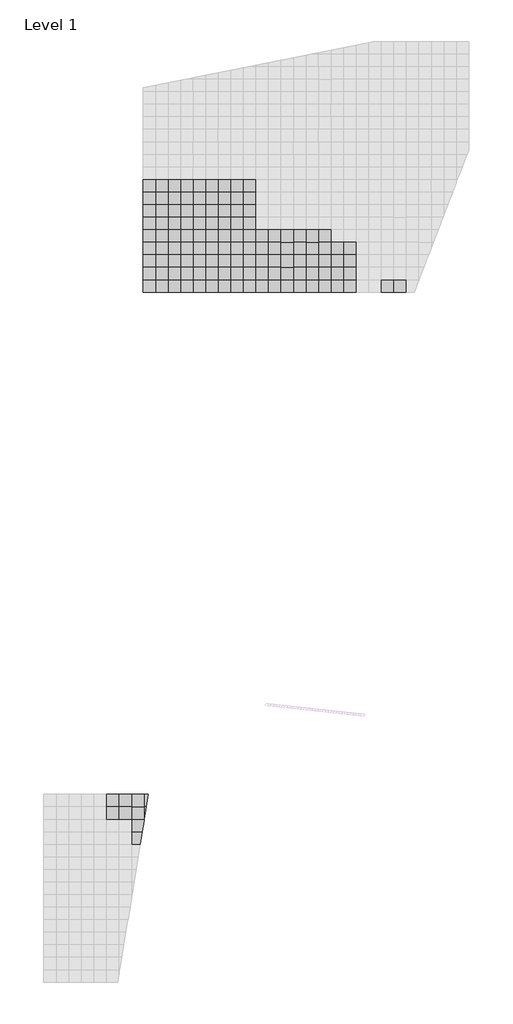
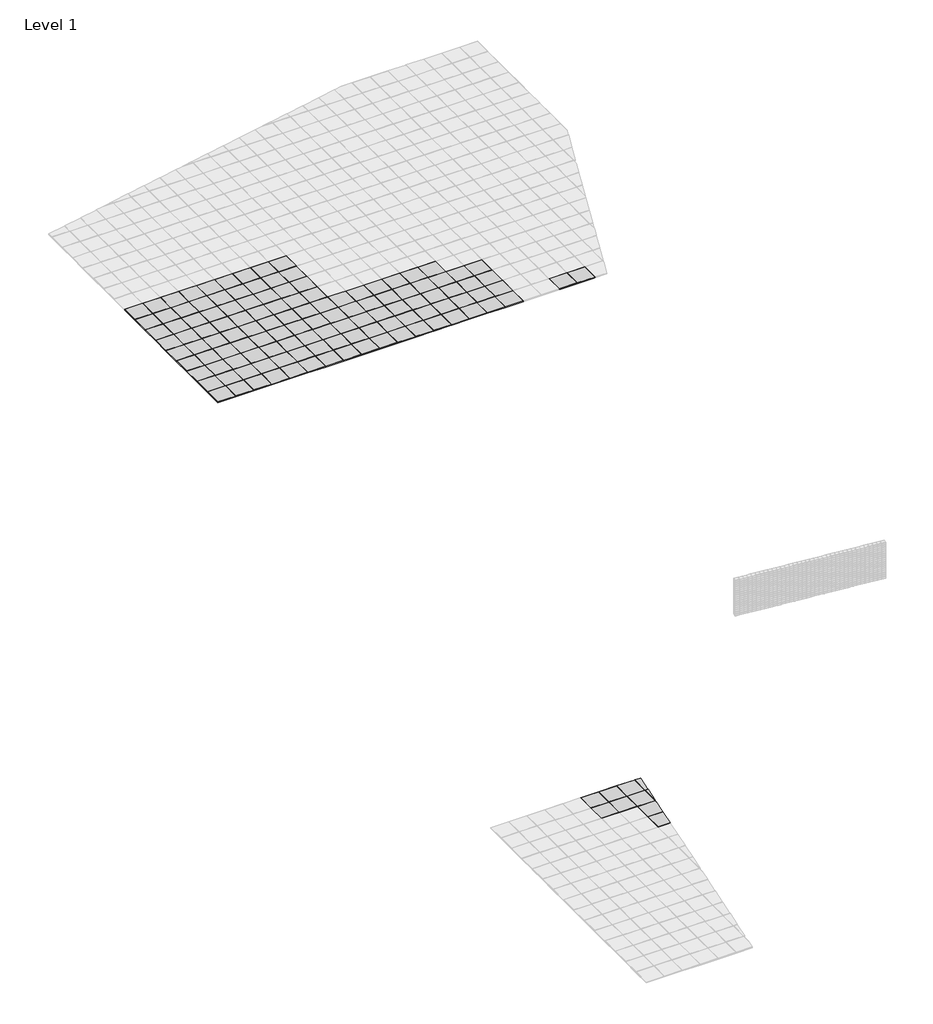
# One storey, part 3 of 18: 131 plates.
"""IFC4 building model written with IfcOpenShell, lengths in millimetres."""

import ifcopenshell
import ifcopenshell.guid

model = None  # the IFC model being written
_history = None  # IfcOwnerHistory: only IFC2X3 demands one
_inside = {}  # id of a spatial element -> (the spatial element, [elements in it])
_under = {}  # id of a project, library or spatial element -> (it, [spatial elements below it])
_declared = {}  # id of a project -> (the project, [libraries it declares])
_typed = {}  # id of a type object -> (the type object, [elements of that type])
_made_of = {}  # id of a material, layer set ... -> (it, [elements and type objects made of it])


def new_model(schema):
    """Start an empty IFC model of exactly this schema.

    Asked for "IFC4X3", IfcOpenShell would pick the latest addendum, in which some entities
    have other attributes; the version numbers below select the first issue.
    IFC2X3 requires an IfcOwnerHistory on every rooted entity: one is made here for all.
    """
    global model, _history
    if schema == "IFC4X3":
        model = ifcopenshell.file(schema_version=(4, 3, 0, 0))
    else:
        model = ifcopenshell.file(schema=schema)
    _inside.clear()
    _under.clear()
    _declared.clear()
    _typed.clear()
    _made_of.clear()
    _history = None
    if model.schema == "IFC2X3":
        org = make("IfcOrganization", Name="unknown")
        user = make(
            "IfcPersonAndOrganization",
            ThePerson=make("IfcPerson", FamilyName="unknown"),
            TheOrganization=org,
        )
        app = make(
            "IfcApplication",
            ApplicationDeveloper=org,
            Version="unknown",
            ApplicationFullName="unknown",
            ApplicationIdentifier="unknown",
        )
        _history = make(
            "IfcOwnerHistory",
            OwningUser=user,
            OwningApplication=app,
            ChangeAction="ADDED",
            CreationDate=0,
        )
    return model


def make(cls, **values):
    """One entity of the class cls with the attributes given. An attribute that is None is left unset."""
    return model.create_entity(
        cls, **{name: value for name, value in values.items() if value is not None}
    )


def rooted(cls, **values):
    """An entity with a GlobalId (a new one), such as an element, a storey or a relation."""
    return make(cls, GlobalId=ifcopenshell.guid.new(), OwnerHistory=_history, **values)


def si_unit(unit_type, name, prefix=None):
    """IfcSIUnit, for example si_unit("LENGTHUNIT", "METRE", prefix="MILLI")."""
    return make("IfcSIUnit", UnitType=unit_type, Prefix=prefix, Name=name)


def assignment(units):
    """IfcUnitAssignment: the units of a project."""
    return None if units is None else make("IfcUnitAssignment", Units=units)


def point(xyz):
    """IfcCartesianPoint."""
    return None if xyz is None else make("IfcCartesianPoint", Coordinates=xyz)


def direction(xyz):
    """IfcDirection."""
    return None if xyz is None else make("IfcDirection", DirectionRatios=xyz)


def frame(location, z_axis=None, x_axis=None):
    """IfcAxis2Placement3D, a coordinate frame: its origin and axes. An axis left out is left unset."""
    return make(
        "IfcAxis2Placement3D",
        Location=point(location),
        Axis=direction(z_axis),
        RefDirection=direction(x_axis),
    )


def origin():
    """The frame at (0, 0, 0) with its axes left unset."""
    return frame((0.0, 0.0, 0.0))


def origin_with_axes():
    """The frame at (0, 0, 0) with the z axis (0, 0, 1) and the x axis (1, 0, 0) written out."""
    return frame((0.0, 0.0, 0.0), z_axis=(0.0, 0.0, 1.0), x_axis=(1.0, 0.0, 0.0))


def place(relative_to, where):
    """IfcLocalPlacement: puts the frame where relative to a parent placement (None: the world)."""
    return make(
        "IfcLocalPlacement", PlacementRelTo=relative_to, RelativePlacement=where
    )


def context(
    kind, dimensions, precision=None, world=None, true_north=None, identifier=None
):
    """IfcGeometricRepresentationContext, for example the 3D "Model" context."""
    return make(
        "IfcGeometricRepresentationContext",
        ContextIdentifier=identifier,
        ContextType=kind,
        CoordinateSpaceDimension=dimensions,
        Precision=precision,
        WorldCoordinateSystem=world,
        TrueNorth=true_north,
    )


def project(units=None, contexts=None):
    """IfcProject with its units and contexts."""
    return rooted(
        "IfcProject",
        Name="project",
        RepresentationContexts=contexts,
        UnitsInContext=assignment(units),
    )


def spatial(cls, under=None, at=None, **own):
    """A site, building, storey or space (cls), placed at a placement, below another one or the project."""
    s = rooted(cls, ObjectPlacement=at, **own)
    if under is not None:
        _under.setdefault(under.id(), (under, []))[1].append(s)
    return s


def polyline(points):
    """IfcPolyline through the points."""
    return make("IfcPolyline", Points=[point(p) for p in points])


def outline(outer, holes=None, kind="AREA"):
    """IfcArbitraryClosedProfileDef: a profile drawn as a closed curve; with holes, ...WithVoids."""
    if holes is None:
        return make("IfcArbitraryClosedProfileDef", ProfileType=kind, OuterCurve=outer)
    return make(
        "IfcArbitraryProfileDefWithVoids",
        ProfileType=kind,
        OuterCurve=outer,
        InnerCurves=holes,
    )


def extrude(swept, where, along, depth):
    """IfcExtrudedAreaSolid: the profile swept, set in the frame where, extruded along a direction by depth."""
    return make(
        "IfcExtrudedAreaSolid",
        SweptArea=swept,
        Position=where,
        ExtrudedDirection=direction(along),
        Depth=depth,
    )


def shape(context_of_items, identifier, shape_type, items):
    """IfcShapeRepresentation: the items that make up one representation, for example the "Body"."""
    return make(
        "IfcShapeRepresentation",
        ContextOfItems=context_of_items,
        RepresentationIdentifier=identifier,
        RepresentationType=shape_type,
        Items=items,
    )


def source(mapping_origin, context_of_items, identifier, shape_type, items):
    """IfcRepresentationMap: a shape defined once, which mapped items show again and again."""
    return make(
        "IfcRepresentationMap",
        MappingOrigin=mapping_origin,
        MappedRepresentation=shape(context_of_items, identifier, shape_type, items),
    )


def transform(
    local_origin,
    x_axis=None,
    y_axis=None,
    z_axis=None,
    scale=None,
    scale2=None,
    scale3=None,
    uniform=True,
):
    """IfcCartesianTransformationOperator3D, or its non-uniform kind. x_axis, y_axis, z_axis: its Axis1, 2, 3."""
    if uniform:
        return make(
            "IfcCartesianTransformationOperator3D",
            Axis1=direction(x_axis),
            Axis2=direction(y_axis),
            LocalOrigin=point(local_origin),
            Scale=scale,
            Axis3=direction(z_axis),
        )
    return make(
        "IfcCartesianTransformationOperator3DnonUniform",
        Axis1=direction(x_axis),
        Axis2=direction(y_axis),
        LocalOrigin=point(local_origin),
        Scale=scale,
        Axis3=direction(z_axis),
        Scale2=scale2,
        Scale3=scale3,
    )


def mapped(mapping_source, mapping_target):
    """IfcMappedItem: shows the shape of a source again, moved by a transform."""
    return make(
        "IfcMappedItem", MappingSource=mapping_source, MappingTarget=mapping_target
    )


def made_of(thing, what):
    """Note that an element or type object is made of a material, layer set ...; save() writes the relation."""
    if what is not None:
        _made_of.setdefault(what.id(), (what, []))[1].append(thing)
    return thing


def element(
    cls,
    number,
    at=None,
    inside=None,
    cuts=None,
    type_object=None,
    material=None,
    context=None,
    identifier="Body",
    shape_type=None,
    held_by="IfcProductDefinitionShape",
    body=None,
    shapes=None,
    **own,
):
    """One element of the class cls, such as IfcWall. Its Tag is "e" and its number.

    at: its placement. inside: the storey or other place that contains it. cuts: it is an
    opening in that element (IfcRelVoidsElement). A single representation is given by context,
    identifier, shape_type and body (its items); several are given by shapes. held_by: the class
    of the entity that holds the representations. save() writes the other relations.
    """
    e = rooted(cls, Tag="e%d" % number, ObjectPlacement=at, **own)
    if body is not None:
        shapes = [shape(context, identifier, shape_type, body)]
    if shapes is not None:
        e.Representation = make(held_by, Representations=shapes)
    if inside is not None:
        _inside.setdefault(inside.id(), (inside, []))[1].append(e)
    if cuts is not None:
        rooted(
            "IfcRelVoidsElement", RelatingBuildingElement=cuts, RelatedOpeningElement=e
        )
    if type_object is not None:
        _typed.setdefault(type_object.id(), (type_object, []))[1].append(e)
    return made_of(e, material)


def aggregate(whole, parts):
    """IfcRelAggregates: a whole, such as a stair, and the parts it consists of."""
    return rooted("IfcRelAggregates", RelatingObject=whole, RelatedObjects=parts)


def save(model, path):
    """Write the relations noted so far, then the file.

    IfcRelAggregates (storeys below a building ...), IfcRelContainedInSpatialStructure (elements
    in a storey), IfcRelDefinesByType, IfcRelAssociatesMaterial and IfcRelDeclares: one each for
    every whole, place, type object, material and project.
    """
    for whole, parts in _under.values():
        aggregate(whole, parts)
    for where, things in _inside.values():
        rooted(
            "IfcRelContainedInSpatialStructure",
            RelatedElements=things,
            RelatingStructure=where,
        )
    for kind, things in _typed.values():
        rooted("IfcRelDefinesByType", RelatedObjects=things, RelatingType=kind)
    for what, things in _made_of.values():
        rooted("IfcRelAssociatesMaterial", RelatedObjects=things, RelatingMaterial=what)
    for by, libraries in _declared.values():
        rooted("IfcRelDeclares", RelatingContext=by, RelatedDefinitions=libraries)
    model.write(path)


def type_1_8eb2385c(model_context):
    return source(origin(), model_context, "Body", "SweptSolid", [
        extrude(outline(polyline([(1000.0, 500.0), (500.0, 500.0), (500.0, 1000.0), (1000.0, 1000.0), (1000.0, 500.0)]), holes=[polyline([(995.0, 995.0), (505.0, 995.0), (505.0, 505.0), (995.0, 505.0), (995.0, 995.0)])]), origin_with_axes(), (0.0, 0.0, 1.0), 18.0),
        extrude(outline(polyline([(505.0, 995.0), (995.0, 995.0), (995.0, 505.0), (505.0, 505.0), (505.0, 995.0)])), origin_with_axes(), (0.0, 0.0, 1.0), 20.0),
    ])


model = new_model("IFC4")

# Units and contexts
model_context = context("Model", 3, world=origin())
ifc_project = project(units=[si_unit("LENGTHUNIT", "METRE", prefix="MILLI")], contexts=[model_context])

# Site, building, storey
site = spatial("IfcSite", under=ifc_project)
building = spatial("IfcBuilding", under=site)
storey = spatial("IfcBuildingStorey", under=building, Name="Level 1", Elevation=0.0)

# Plates
placement = place(None, origin())
element("IfcPlate", 1, ObjectType="00_CPA_tegel : Type 1", at=placement, inside=storey, context=model_context, shape_type="SweptSolid", body=[
    extrude(outline(polyline([(3554.3495497, -9904.4739057), (3554.3593325, -9414.4739058), (3972.5227781, -9414.4822543), (3892.8479077, -9904.4806637), (3554.3495497, -9904.4739057)])), frame((0.0, 0.0, 1000.0), z_axis=(0.0, 0.0, 1.0), x_axis=(1.0, 0.0, 0.0)), (0.0, 0.0, 1.0), 20.0),
    extrude(outline(polyline([(3549.3494499, -9909.4738058), (3549.3594323, -9409.4738059), (3973.335787, -9409.4822706), (3972.5227781, -9414.4822543), (3554.3593325, -9414.4739058), (3554.3495497, -9904.4739057), (3892.8479077, -9904.4806637), (3892.0348989, -9909.4806475), (3549.3494499, -9909.4738058)])), frame((0.0, 0.0, 1000.0), z_axis=(0.0, 0.0, 1.0), x_axis=(1.0, 0.0, 0.0)), (0.0, 0.0, 1.0), 18.0),
])
element("IfcPlate", 2, ObjectType="00_CPA_tegel : Type 1", at=placement, inside=storey, context=model_context, shape_type="SweptSolid", body=[
    extrude(outline(polyline([(3554.3595321, -9404.4739058), (3554.3693149, -8914.4739059), (4044.3693148, -8914.4836887), (4044.3681538, -8972.6350365), (3974.1487959, -9404.4822868), (3554.3595321, -9404.4739058)])), frame((0.0, 0.0, 1000.0), z_axis=(0.0, 0.0, 1.0), x_axis=(1.0, 0.0, 0.0)), (0.0, 0.0, 1.0), 20.0),
    extrude(outline(polyline([(3549.3694147, -8909.473806), (4049.3694146, -8909.4837885), (4049.3687678, -8941.8813887), (4044.3681538, -8972.6350365), (4044.3693148, -8914.4836887), (3554.3693149, -8914.4739059), (3554.3595321, -9404.4739058), (3974.1487959, -9404.4822868), (3973.335787, -9409.4822706), (3549.3594323, -9409.4738059), (3549.3694147, -8909.473806)])), frame((0.0, 0.0, 1000.0), z_axis=(0.0, 0.0, 1.0), x_axis=(1.0, 0.0, 0.0)), (0.0, 0.0, 1.0), 18.0),
])
element("IfcPlate", 3, ObjectType="00_CPA_tegel : Type 1", at=placement, inside=storey, context=model_context, shape_type="SweptSolid", body=[
    extrude(outline(polyline([(3554.3695146, -8904.4739059), (3554.3792973, -8414.473906), (4044.3792972, -8414.4836888), (4044.3695145, -8904.4836887), (3554.3695146, -8904.4739059)])), frame((0.0, 0.0, 1000.0), z_axis=(0.0, 0.0, 1.0), x_axis=(1.0, 0.0, 0.0)), (0.0, 0.0, 1.0), 20.0),
    extrude(outline(polyline([(4049.3694146, -8909.4837885), (3549.3694147, -8909.473806), (3549.3793972, -8409.4738061), (4049.3793971, -8409.4837886), (4049.3694146, -8909.4837885)]), holes=[polyline([(4044.3792972, -8414.4836888), (3554.3792973, -8414.473906), (3554.3695146, -8904.4739059), (4044.3695145, -8904.4836887), (4044.3792972, -8414.4836888)])]), frame((0.0, 0.0, 1000.0), z_axis=(0.0, 0.0, 1.0), x_axis=(1.0, 0.0, 0.0)), (0.0, 0.0, 1.0), 18.0),
])
element("IfcPlate", 4, ObjectType="00_CPA_tegel : Type 1", at=placement, inside=storey, context=model_context, shape_type="SweptSolid", body=[
    extrude(outline(polyline([(4054.3695145, -8904.4838883), (4054.3792972, -8414.4838884), (4135.1245544, -8414.4855005), (4055.4496841, -8904.4839099), (4054.3695145, -8904.4838883)])), frame((0.0, 0.0, 1000.0), z_axis=(0.0, 0.0, 1.0), x_axis=(1.0, 0.0, 0.0)), (0.0, 0.0, 1.0), 20.0),
    extrude(outline(polyline([(4049.3694146, -8909.4837885), (4049.3793971, -8409.4837886), (4135.9375633, -8409.4855167), (4135.1245544, -8414.4855005), (4054.3792972, -8414.4838884), (4054.3695145, -8904.4838883), (4055.4496841, -8904.4839099), (4054.6366752, -8909.4838936), (4049.3694146, -8909.4837885)])), frame((0.0, 0.0, 1000.0), z_axis=(0.0, 0.0, 1.0), x_axis=(1.0, 0.0, 0.0)), (0.0, 0.0, 1.0), 18.0),
])
element("IfcPlate", 5, ObjectType="00_CPA_tegel : Type 1", at=placement, inside=storey, context=model_context, shape_type="SweptSolid", body=[
    extrude(outline(polyline([(4054.3794969, -8404.4838884), (4054.3892797, -7914.4838885), (4216.4254426, -7914.4871235), (4136.7505722, -8404.4855329), (4054.3794969, -8404.4838884)])), frame((0.0, 0.0, 1000.0), z_axis=(0.0, 0.0, 1.0), x_axis=(1.0, 0.0, 0.0)), (0.0, 0.0, 1.0), 20.0),
    extrude(outline(polyline([(4049.3793971, -8409.4837886), (4049.3893795, -7909.4837887), (4217.2384514, -7909.4871398), (4216.4254426, -7914.4871235), (4054.3892797, -7914.4838885), (4054.3794969, -8404.4838884), (4136.7505722, -8404.4855329), (4135.9375633, -8409.4855167), (4049.3793971, -8409.4837886)])), frame((0.0, 0.0, 1000.0), z_axis=(0.0, 0.0, 1.0), x_axis=(1.0, 0.0, 0.0)), (0.0, 0.0, 1.0), 18.0),
])
type_1_shape = type_1_8eb2385c(model_context)
element("IfcPlate", 6, ObjectType="00_CPA_tegel : Type 1", at=placement, inside=storey, context=model_context, shape_type="MappedRepresentation", body=[
    mapped(type_1_shape, transform((3506.2147669, 11592.7016515, 0.0), x_axis=(1.0000000000000002, 0.0, 0.0), y_axis=(0.0, 1.0000000000000002, 0.0), z_axis=(0.0, 0.0, 1.0))),
])
element("IfcPlate", 7, ObjectType="00_CPA_tegel : Type 1", at=placement, inside=storey, context=model_context, shape_type="MappedRepresentation", body=[
    mapped(type_1_shape, transform((4006.2147669, 11592.7016515, 0.0), x_axis=(1.0000000000000002, 0.0, 0.0), y_axis=(0.0, 1.0000000000000002, 0.0), z_axis=(0.0, 0.0, 1.0))),
])
element("IfcPlate", 8, ObjectType="00_CPA_tegel : Type 1", at=placement, inside=storey, context=model_context, shape_type="MappedRepresentation", body=[
    mapped(type_1_shape, transform((4506.2147669, 11592.7016515, 0.0), x_axis=(1.0000000000000002, 0.0, 0.0), y_axis=(0.0, 1.0000000000000002, 0.0), z_axis=(0.0, 0.0, 1.0))),
])
element("IfcPlate", 9, ObjectType="00_CPA_tegel : Type 1", at=placement, inside=storey, context=model_context, shape_type="MappedRepresentation", body=[
    mapped(type_1_shape, transform((5006.2147669, 11592.7016515, 0.0), x_axis=(1.0000000000000002, 0.0, 0.0), y_axis=(0.0, 1.0000000000000002, 0.0), z_axis=(0.0, 0.0, 1.0))),
])
element("IfcPlate", 10, ObjectType="00_CPA_tegel : Type 1", at=placement, inside=storey, context=model_context, shape_type="MappedRepresentation", body=[
    mapped(type_1_shape, transform((5506.2147669, 11592.7016515, 0.0), x_axis=(1.0000000000000002, 0.0, 0.0), y_axis=(0.0, 1.0000000000000002, 0.0), z_axis=(0.0, 0.0, 1.0))),
])
element("IfcPlate", 11, ObjectType="00_CPA_tegel : Type 1", at=placement, inside=storey, context=model_context, shape_type="MappedRepresentation", body=[
    mapped(type_1_shape, transform((6006.2147669, 11592.7016515, 0.0), x_axis=(1.0000000000000002, 0.0, 0.0), y_axis=(0.0, 1.0000000000000002, 0.0), z_axis=(0.0, 0.0, 1.0))),
])
element("IfcPlate", 12, ObjectType="00_CPA_tegel : Type 1", at=placement, inside=storey, context=model_context, shape_type="MappedRepresentation", body=[
    mapped(type_1_shape, transform((6506.2147669, 11592.7016515, 0.0), x_axis=(1.0000000000000002, 0.0, 0.0), y_axis=(0.0, 1.0000000000000002, 0.0), z_axis=(0.0, 0.0, 1.0))),
])
element("IfcPlate", 13, ObjectType="00_CPA_tegel : Type 1", at=placement, inside=storey, context=model_context, shape_type="MappedRepresentation", body=[
    mapped(type_1_shape, transform((7006.2147669, 11592.7016515, 0.0), x_axis=(1.0000000000000002, 0.0, 0.0), y_axis=(0.0, 1.0000000000000002, 0.0), z_axis=(0.0, 0.0, 1.0))),
])
element("IfcPlate", 14, ObjectType="00_CPA_tegel : Type 1", at=placement, inside=storey, context=model_context, shape_type="MappedRepresentation", body=[
    mapped(type_1_shape, transform((7506.2147669, 11592.7016515, 0.0), x_axis=(1.0000000000000002, 0.0, 0.0), y_axis=(0.0, 1.0000000000000002, 0.0), z_axis=(0.0, 0.0, 1.0))),
])
element("IfcPlate", 15, ObjectType="00_CPA_tegel : Type 1", at=placement, inside=storey, context=model_context, shape_type="MappedRepresentation", body=[
    mapped(type_1_shape, transform((3506.2147669, 12092.7016515, 0.0), x_axis=(1.0000000000000002, 0.0, 0.0), y_axis=(0.0, 1.0000000000000002, 0.0), z_axis=(0.0, 0.0, 1.0))),
])
element("IfcPlate", 16, ObjectType="00_CPA_tegel : Type 1", at=placement, inside=storey, context=model_context, shape_type="MappedRepresentation", body=[
    mapped(type_1_shape, transform((4006.2147669, 12092.7016515, 0.0), x_axis=(1.0000000000000002, 0.0, 0.0), y_axis=(0.0, 1.0000000000000002, 0.0), z_axis=(0.0, 0.0, 1.0))),
])
element("IfcPlate", 17, ObjectType="00_CPA_tegel : Type 1", at=placement, inside=storey, context=model_context, shape_type="MappedRepresentation", body=[
    mapped(type_1_shape, transform((4506.2147669, 12092.7016515, 0.0), x_axis=(1.0000000000000002, 0.0, 0.0), y_axis=(0.0, 1.0000000000000002, 0.0), z_axis=(0.0, 0.0, 1.0))),
])
element("IfcPlate", 18, ObjectType="00_CPA_tegel : Type 1", at=placement, inside=storey, context=model_context, shape_type="MappedRepresentation", body=[
    mapped(type_1_shape, transform((5006.2147669, 12092.7016515, 0.0), x_axis=(1.0000000000000002, 0.0, 0.0), y_axis=(0.0, 1.0000000000000002, 0.0), z_axis=(0.0, 0.0, 1.0))),
])
element("IfcPlate", 19, ObjectType="00_CPA_tegel : Type 1", at=placement, inside=storey, context=model_context, shape_type="MappedRepresentation", body=[
    mapped(type_1_shape, transform((5506.2147669, 12092.7016515, 0.0), x_axis=(1.0000000000000002, 0.0, 0.0), y_axis=(0.0, 1.0000000000000002, 0.0), z_axis=(0.0, 0.0, 1.0))),
])
element("IfcPlate", 20, ObjectType="00_CPA_tegel : Type 1", at=placement, inside=storey, context=model_context, shape_type="MappedRepresentation", body=[
    mapped(type_1_shape, transform((6006.2147669, 12092.7016515, 0.0), x_axis=(1.0000000000000002, 0.0, 0.0), y_axis=(0.0, 1.0000000000000002, 0.0), z_axis=(0.0, 0.0, 1.0))),
])
element("IfcPlate", 21, ObjectType="00_CPA_tegel : Type 1", at=placement, inside=storey, context=model_context, shape_type="MappedRepresentation", body=[
    mapped(type_1_shape, transform((6506.2147669, 12092.7016515, 0.0), x_axis=(1.0000000000000002, 0.0, 0.0), y_axis=(0.0, 1.0000000000000002, 0.0), z_axis=(0.0, 0.0, 1.0))),
])
element("IfcPlate", 22, ObjectType="00_CPA_tegel : Type 1", at=placement, inside=storey, context=model_context, shape_type="MappedRepresentation", body=[
    mapped(type_1_shape, transform((7006.2147669, 12092.7016515, 0.0), x_axis=(1.0000000000000002, 0.0, 0.0), y_axis=(0.0, 1.0000000000000002, 0.0), z_axis=(0.0, 0.0, 1.0))),
])
element("IfcPlate", 23, ObjectType="00_CPA_tegel : Type 1", at=placement, inside=storey, context=model_context, shape_type="MappedRepresentation", body=[
    mapped(type_1_shape, transform((7506.2147669, 12092.7016515, 0.0), x_axis=(1.0000000000000002, 0.0, 0.0), y_axis=(0.0, 1.0000000000000002, 0.0), z_axis=(0.0, 0.0, 1.0))),
])
element("IfcPlate", 24, ObjectType="00_CPA_tegel : Type 1", at=placement, inside=storey, context=model_context, shape_type="MappedRepresentation", body=[
    mapped(type_1_shape, transform((3506.2147669, 12592.7016515, 0.0), x_axis=(1.0000000000000002, 0.0, 0.0), y_axis=(0.0, 1.0000000000000002, 0.0), z_axis=(0.0, 0.0, 1.0))),
])
element("IfcPlate", 25, ObjectType="00_CPA_tegel : Type 1", at=placement, inside=storey, context=model_context, shape_type="MappedRepresentation", body=[
    mapped(type_1_shape, transform((4006.2147669, 12592.7016515, 0.0), x_axis=(1.0000000000000002, 0.0, 0.0), y_axis=(0.0, 1.0000000000000002, 0.0), z_axis=(0.0, 0.0, 1.0))),
])
element("IfcPlate", 26, ObjectType="00_CPA_tegel : Type 1", at=placement, inside=storey, context=model_context, shape_type="MappedRepresentation", body=[
    mapped(type_1_shape, transform((4506.2147669, 12592.7016515, 0.0), x_axis=(1.0000000000000002, 0.0, 0.0), y_axis=(0.0, 1.0000000000000002, 0.0), z_axis=(0.0, 0.0, 1.0))),
])
element("IfcPlate", 27, ObjectType="00_CPA_tegel : Type 1", at=placement, inside=storey, context=model_context, shape_type="MappedRepresentation", body=[
    mapped(type_1_shape, transform((5006.2147669, 12592.7016515, 0.0), x_axis=(1.0000000000000002, 0.0, 0.0), y_axis=(0.0, 1.0000000000000002, 0.0), z_axis=(0.0, 0.0, 1.0))),
])
element("IfcPlate", 28, ObjectType="00_CPA_tegel : Type 1", at=placement, inside=storey, context=model_context, shape_type="MappedRepresentation", body=[
    mapped(type_1_shape, transform((5506.2147669, 12592.7016515, 0.0), x_axis=(1.0000000000000002, 0.0, 0.0), y_axis=(0.0, 1.0000000000000002, 0.0), z_axis=(0.0, 0.0, 1.0))),
])
element("IfcPlate", 29, ObjectType="00_CPA_tegel : Type 1", at=placement, inside=storey, context=model_context, shape_type="MappedRepresentation", body=[
    mapped(type_1_shape, transform((6006.2147669, 12592.7016515, 0.0), x_axis=(1.0000000000000002, 0.0, 0.0), y_axis=(0.0, 1.0000000000000002, 0.0), z_axis=(0.0, 0.0, 1.0))),
])
element("IfcPlate", 30, ObjectType="00_CPA_tegel : Type 1", at=placement, inside=storey, context=model_context, shape_type="MappedRepresentation", body=[
    mapped(type_1_shape, transform((6506.2147669, 12592.7016515, 0.0), x_axis=(1.0000000000000002, 0.0, 0.0), y_axis=(0.0, 1.0000000000000002, 0.0), z_axis=(0.0, 0.0, 1.0))),
])
element("IfcPlate", 31, ObjectType="00_CPA_tegel : Type 1", at=placement, inside=storey, context=model_context, shape_type="MappedRepresentation", body=[
    mapped(type_1_shape, transform((7006.2147669, 12592.7016515, 0.0), x_axis=(1.0000000000000002, 0.0, 0.0), y_axis=(0.0, 1.0000000000000002, 0.0), z_axis=(0.0, 0.0, 1.0))),
])
element("IfcPlate", 32, ObjectType="00_CPA_tegel : Type 1", at=placement, inside=storey, context=model_context, shape_type="MappedRepresentation", body=[
    mapped(type_1_shape, transform((7506.2147669, 12592.7016515, 0.0), x_axis=(1.0000000000000002, 0.0, 0.0), y_axis=(0.0, 1.0000000000000002, 0.0), z_axis=(0.0, 0.0, 1.0))),
])
element("IfcPlate", 33, ObjectType="00_CPA_tegel : Type 1", at=placement, inside=storey, context=model_context, shape_type="MappedRepresentation", body=[
    mapped(type_1_shape, transform((3506.2147669, 13092.7016515, 0.0), x_axis=(1.0000000000000002, 0.0, 0.0), y_axis=(0.0, 1.0000000000000002, 0.0), z_axis=(0.0, 0.0, 1.0))),
])
element("IfcPlate", 34, ObjectType="00_CPA_tegel : Type 1", at=placement, inside=storey, context=model_context, shape_type="MappedRepresentation", body=[
    mapped(type_1_shape, transform((4006.2147669, 13092.7016515, 0.0), x_axis=(1.0000000000000002, 0.0, 0.0), y_axis=(0.0, 1.0000000000000002, 0.0), z_axis=(0.0, 0.0, 1.0))),
])
element("IfcPlate", 35, ObjectType="00_CPA_tegel : Type 1", at=placement, inside=storey, context=model_context, shape_type="MappedRepresentation", body=[
    mapped(type_1_shape, transform((4506.2147669, 13092.7016515, 0.0), x_axis=(1.0000000000000002, 0.0, 0.0), y_axis=(0.0, 1.0000000000000002, 0.0), z_axis=(0.0, 0.0, 1.0))),
])
element("IfcPlate", 36, ObjectType="00_CPA_tegel : Type 1", at=placement, inside=storey, context=model_context, shape_type="MappedRepresentation", body=[
    mapped(type_1_shape, transform((5006.2147669, 13092.7016515, 0.0), x_axis=(1.0000000000000002, 0.0, 0.0), y_axis=(0.0, 1.0000000000000002, 0.0), z_axis=(0.0, 0.0, 1.0))),
])
element("IfcPlate", 37, ObjectType="00_CPA_tegel : Type 1", at=placement, inside=storey, context=model_context, shape_type="MappedRepresentation", body=[
    mapped(type_1_shape, transform((5506.2147669, 13092.7016515, 0.0), x_axis=(1.0000000000000002, 0.0, 0.0), y_axis=(0.0, 1.0000000000000002, 0.0), z_axis=(0.0, 0.0, 1.0))),
])
element("IfcPlate", 38, ObjectType="00_CPA_tegel : Type 1", at=placement, inside=storey, context=model_context, shape_type="MappedRepresentation", body=[
    mapped(type_1_shape, transform((6006.2147669, 13092.7016515, 0.0), x_axis=(1.0000000000000002, 0.0, 0.0), y_axis=(0.0, 1.0000000000000002, 0.0), z_axis=(0.0, 0.0, 1.0))),
])
element("IfcPlate", 39, ObjectType="00_CPA_tegel : Type 1", at=placement, inside=storey, context=model_context, shape_type="MappedRepresentation", body=[
    mapped(type_1_shape, transform((6506.2147669, 13092.7016515, 0.0), x_axis=(1.0000000000000002, 0.0, 0.0), y_axis=(0.0, 1.0000000000000002, 0.0), z_axis=(0.0, 0.0, 1.0))),
])
element("IfcPlate", 40, ObjectType="00_CPA_tegel : Type 1", at=placement, inside=storey, context=model_context, shape_type="MappedRepresentation", body=[
    mapped(type_1_shape, transform((7006.2147669, 13092.7016515, 0.0), x_axis=(1.0000000000000002, 0.0, 0.0), y_axis=(0.0, 1.0000000000000002, 0.0), z_axis=(0.0, 0.0, 1.0))),
])
element("IfcPlate", 41, ObjectType="00_CPA_tegel : Type 1", at=placement, inside=storey, context=model_context, shape_type="MappedRepresentation", body=[
    mapped(type_1_shape, transform((7506.2147669, 13092.7016515, 0.0), x_axis=(1.0000000000000002, 0.0, 0.0), y_axis=(0.0, 1.0000000000000002, 0.0), z_axis=(0.0, 0.0, 1.0))),
])
element("IfcPlate", 42, ObjectType="00_CPA_tegel : Type 1", at=placement, inside=storey, context=model_context, shape_type="MappedRepresentation", body=[
    mapped(type_1_shape, transform((3506.2147669, 13592.7016515, 0.0), x_axis=(1.0000000000000002, 0.0, 0.0), y_axis=(0.0, 1.0000000000000002, 0.0), z_axis=(0.0, 0.0, 1.0))),
])
element("IfcPlate", 43, ObjectType="00_CPA_tegel : Type 1", at=placement, inside=storey, context=model_context, shape_type="MappedRepresentation", body=[
    mapped(type_1_shape, transform((4006.2147669, 13592.7016515, 0.0), x_axis=(1.0000000000000002, 0.0, 0.0), y_axis=(0.0, 1.0000000000000002, 0.0), z_axis=(0.0, 0.0, 1.0))),
])
element("IfcPlate", 44, ObjectType="00_CPA_tegel : Type 1", at=placement, inside=storey, context=model_context, shape_type="MappedRepresentation", body=[
    mapped(type_1_shape, transform((4506.2147669, 13592.7016515, 0.0), x_axis=(1.0000000000000002, 0.0, 0.0), y_axis=(0.0, 1.0000000000000002, 0.0), z_axis=(0.0, 0.0, 1.0))),
])
element("IfcPlate", 45, ObjectType="00_CPA_tegel : Type 1", at=placement, inside=storey, context=model_context, shape_type="MappedRepresentation", body=[
    mapped(type_1_shape, transform((5006.2147669, 13592.7016515, 0.0), x_axis=(1.0000000000000002, 0.0, 0.0), y_axis=(0.0, 1.0000000000000002, 0.0), z_axis=(0.0, 0.0, 1.0))),
])
element("IfcPlate", 46, ObjectType="00_CPA_tegel : Type 1", at=placement, inside=storey, context=model_context, shape_type="MappedRepresentation", body=[
    mapped(type_1_shape, transform((5506.2147669, 13592.7016515, 0.0), x_axis=(1.0000000000000002, 0.0, 0.0), y_axis=(0.0, 1.0000000000000002, 0.0), z_axis=(0.0, 0.0, 1.0))),
])
element("IfcPlate", 47, ObjectType="00_CPA_tegel : Type 1", at=placement, inside=storey, context=model_context, shape_type="MappedRepresentation", body=[
    mapped(type_1_shape, transform((6006.2147669, 13592.7016515, 0.0), x_axis=(1.0000000000000002, 0.0, 0.0), y_axis=(0.0, 1.0000000000000002, 0.0), z_axis=(0.0, 0.0, 1.0))),
])
element("IfcPlate", 48, ObjectType="00_CPA_tegel : Type 1", at=placement, inside=storey, context=model_context, shape_type="MappedRepresentation", body=[
    mapped(type_1_shape, transform((6506.2147669, 13592.7016515, 0.0), x_axis=(1.0000000000000002, 0.0, 0.0), y_axis=(0.0, 1.0000000000000002, 0.0), z_axis=(0.0, 0.0, 1.0))),
])
element("IfcPlate", 49, ObjectType="00_CPA_tegel : Type 1", at=placement, inside=storey, context=model_context, shape_type="MappedRepresentation", body=[
    mapped(type_1_shape, transform((7006.2147669, 13592.7016515, 0.0), x_axis=(1.0000000000000002, 0.0, 0.0), y_axis=(0.0, 1.0000000000000002, 0.0), z_axis=(0.0, 0.0, 1.0))),
])
element("IfcPlate", 50, ObjectType="00_CPA_tegel : Type 1", at=placement, inside=storey, context=model_context, shape_type="MappedRepresentation", body=[
    mapped(type_1_shape, transform((7506.2147669, 13592.7016515, 0.0), x_axis=(1.0000000000000002, 0.0, 0.0), y_axis=(0.0, 1.0000000000000002, 0.0), z_axis=(0.0, 0.0, 1.0))),
])
element("IfcPlate", 51, ObjectType="00_CPA_tegel : Type 1", at=placement, inside=storey, context=model_context, shape_type="MappedRepresentation", body=[
    mapped(type_1_shape, transform((3506.2147669, 14092.7016515, 0.0), x_axis=(1.0000000000000002, 0.0, 0.0), y_axis=(0.0, 1.0000000000000002, 0.0), z_axis=(0.0, 0.0, 1.0))),
])
element("IfcPlate", 52, ObjectType="00_CPA_tegel : Type 1", at=placement, inside=storey, context=model_context, shape_type="MappedRepresentation", body=[
    mapped(type_1_shape, transform((4006.2147669, 14092.7016515, 0.0), x_axis=(1.0000000000000002, 0.0, 0.0), y_axis=(0.0, 1.0000000000000002, 0.0), z_axis=(0.0, 0.0, 1.0))),
])
element("IfcPlate", 53, ObjectType="00_CPA_tegel : Type 1", at=placement, inside=storey, context=model_context, shape_type="MappedRepresentation", body=[
    mapped(type_1_shape, transform((4506.2147669, 14092.7016515, 0.0), x_axis=(1.0000000000000002, 0.0, 0.0), y_axis=(0.0, 1.0000000000000002, 0.0), z_axis=(0.0, 0.0, 1.0))),
])
element("IfcPlate", 54, ObjectType="00_CPA_tegel : Type 1", at=placement, inside=storey, context=model_context, shape_type="MappedRepresentation", body=[
    mapped(type_1_shape, transform((5006.2147669, 14092.7016515, 0.0), x_axis=(1.0000000000000002, 0.0, 0.0), y_axis=(0.0, 1.0000000000000002, 0.0), z_axis=(0.0, 0.0, 1.0))),
])
element("IfcPlate", 55, ObjectType="00_CPA_tegel : Type 1", at=placement, inside=storey, context=model_context, shape_type="MappedRepresentation", body=[
    mapped(type_1_shape, transform((5506.2147669, 14092.7016515, 0.0), x_axis=(1.0000000000000002, 0.0, 0.0), y_axis=(0.0, 1.0000000000000002, 0.0), z_axis=(0.0, 0.0, 1.0))),
])
element("IfcPlate", 56, ObjectType="00_CPA_tegel : Type 1", at=placement, inside=storey, context=model_context, shape_type="MappedRepresentation", body=[
    mapped(type_1_shape, transform((6006.2147669, 14092.7016515, 0.0), x_axis=(1.0000000000000002, 0.0, 0.0), y_axis=(0.0, 1.0000000000000002, 0.0), z_axis=(0.0, 0.0, 1.0))),
])
element("IfcPlate", 57, ObjectType="00_CPA_tegel : Type 1", at=placement, inside=storey, context=model_context, shape_type="MappedRepresentation", body=[
    mapped(type_1_shape, transform((6506.2147669, 14092.7016515, 0.0), x_axis=(1.0000000000000002, 0.0, 0.0), y_axis=(0.0, 1.0000000000000002, 0.0), z_axis=(0.0, 0.0, 1.0))),
])
element("IfcPlate", 58, ObjectType="00_CPA_tegel : Type 1", at=placement, inside=storey, context=model_context, shape_type="MappedRepresentation", body=[
    mapped(type_1_shape, transform((7006.2147669, 14092.7016515, 0.0), x_axis=(1.0000000000000002, 0.0, 0.0), y_axis=(0.0, 1.0000000000000002, 0.0), z_axis=(0.0, 0.0, 1.0))),
])
element("IfcPlate", 59, ObjectType="00_CPA_tegel : Type 1", at=placement, inside=storey, context=model_context, shape_type="MappedRepresentation", body=[
    mapped(type_1_shape, transform((7506.2147669, 14092.7016515, 0.0), x_axis=(1.0000000000000002, 0.0, 0.0), y_axis=(0.0, 1.0000000000000002, 0.0), z_axis=(0.0, 0.0, 1.0))),
])
element("IfcPlate", 60, ObjectType="00_CPA_tegel : Type 1", at=placement, inside=storey, context=model_context, shape_type="MappedRepresentation", body=[
    mapped(type_1_shape, transform((3506.2147669, 14592.7016515, 0.0), x_axis=(1.0000000000000002, 0.0, 0.0), y_axis=(0.0, 1.0000000000000002, 0.0), z_axis=(0.0, 0.0, 1.0))),
])
element("IfcPlate", 61, ObjectType="00_CPA_tegel : Type 1", at=placement, inside=storey, context=model_context, shape_type="MappedRepresentation", body=[
    mapped(type_1_shape, transform((4006.2147669, 14592.7016515, 0.0), x_axis=(1.0000000000000002, 0.0, 0.0), y_axis=(0.0, 1.0000000000000002, 0.0), z_axis=(0.0, 0.0, 1.0))),
])
element("IfcPlate", 62, ObjectType="00_CPA_tegel : Type 1", at=placement, inside=storey, context=model_context, shape_type="MappedRepresentation", body=[
    mapped(type_1_shape, transform((4506.2147669, 14592.7016515, 0.0), x_axis=(1.0000000000000002, 0.0, 0.0), y_axis=(0.0, 1.0000000000000002, 0.0), z_axis=(0.0, 0.0, 1.0))),
])
element("IfcPlate", 63, ObjectType="00_CPA_tegel : Type 1", at=placement, inside=storey, context=model_context, shape_type="MappedRepresentation", body=[
    mapped(type_1_shape, transform((5006.2147669, 14592.7016515, 0.0), x_axis=(1.0000000000000002, 0.0, 0.0), y_axis=(0.0, 1.0000000000000002, 0.0), z_axis=(0.0, 0.0, 1.0))),
])
element("IfcPlate", 64, ObjectType="00_CPA_tegel : Type 1", at=placement, inside=storey, context=model_context, shape_type="MappedRepresentation", body=[
    mapped(type_1_shape, transform((5506.2147669, 14592.7016515, 0.0), x_axis=(1.0000000000000002, 0.0, 0.0), y_axis=(0.0, 1.0000000000000002, 0.0), z_axis=(0.0, 0.0, 1.0))),
])
element("IfcPlate", 65, ObjectType="00_CPA_tegel : Type 1", at=placement, inside=storey, context=model_context, shape_type="MappedRepresentation", body=[
    mapped(type_1_shape, transform((6006.2147669, 14592.7016515, 0.0), x_axis=(1.0000000000000002, 0.0, 0.0), y_axis=(0.0, 1.0000000000000002, 0.0), z_axis=(0.0, 0.0, 1.0))),
])
element("IfcPlate", 66, ObjectType="00_CPA_tegel : Type 1", at=placement, inside=storey, context=model_context, shape_type="MappedRepresentation", body=[
    mapped(type_1_shape, transform((6506.2147669, 14592.7016515, 0.0), x_axis=(1.0000000000000002, 0.0, 0.0), y_axis=(0.0, 1.0000000000000002, 0.0), z_axis=(0.0, 0.0, 1.0))),
])
element("IfcPlate", 67, ObjectType="00_CPA_tegel : Type 1", at=placement, inside=storey, context=model_context, shape_type="MappedRepresentation", body=[
    mapped(type_1_shape, transform((7006.2147669, 14592.7016515, 0.0), x_axis=(1.0000000000000002, 0.0, 0.0), y_axis=(0.0, 1.0000000000000002, 0.0), z_axis=(0.0, 0.0, 1.0))),
])
element("IfcPlate", 68, ObjectType="00_CPA_tegel : Type 1", at=placement, inside=storey, context=model_context, shape_type="MappedRepresentation", body=[
    mapped(type_1_shape, transform((7506.2147669, 14592.7016515, 0.0), x_axis=(1.0000000000000002, 0.0, 0.0), y_axis=(0.0, 1.0000000000000002, 0.0), z_axis=(0.0, 0.0, 1.0))),
])
element("IfcPlate", 69, ObjectType="00_CPA_tegel : Type 1", at=placement, inside=storey, context=model_context, shape_type="MappedRepresentation", body=[
    mapped(type_1_shape, transform((3506.2147669, 15092.7016515, 0.0), x_axis=(1.0000000000000002, 0.0, 0.0), y_axis=(0.0, 1.0000000000000002, 0.0), z_axis=(0.0, 0.0, 1.0))),
])
element("IfcPlate", 70, ObjectType="00_CPA_tegel : Type 1", at=placement, inside=storey, context=model_context, shape_type="MappedRepresentation", body=[
    mapped(type_1_shape, transform((4006.2147669, 15092.7016515, 0.0), x_axis=(1.0000000000000002, 0.0, 0.0), y_axis=(0.0, 1.0000000000000002, 0.0), z_axis=(0.0, 0.0, 1.0))),
])
element("IfcPlate", 71, ObjectType="00_CPA_tegel : Type 1", at=placement, inside=storey, context=model_context, shape_type="MappedRepresentation", body=[
    mapped(type_1_shape, transform((4506.2147669, 15092.7016515, 0.0), x_axis=(1.0000000000000002, 0.0, 0.0), y_axis=(0.0, 1.0000000000000002, 0.0), z_axis=(0.0, 0.0, 1.0))),
])
element("IfcPlate", 72, ObjectType="00_CPA_tegel : Type 1", at=placement, inside=storey, context=model_context, shape_type="MappedRepresentation", body=[
    mapped(type_1_shape, transform((5006.2147669, 15092.7016515, 0.0), x_axis=(1.0000000000000002, 0.0, 0.0), y_axis=(0.0, 1.0000000000000002, 0.0), z_axis=(0.0, 0.0, 1.0))),
])
element("IfcPlate", 73, ObjectType="00_CPA_tegel : Type 1", at=placement, inside=storey, context=model_context, shape_type="MappedRepresentation", body=[
    mapped(type_1_shape, transform((5506.2147669, 15092.7016515, 0.0), x_axis=(1.0000000000000002, 0.0, 0.0), y_axis=(0.0, 1.0000000000000002, 0.0), z_axis=(0.0, 0.0, 1.0))),
])
element("IfcPlate", 74, ObjectType="00_CPA_tegel : Type 1", at=placement, inside=storey, context=model_context, shape_type="MappedRepresentation", body=[
    mapped(type_1_shape, transform((6006.2147669, 15092.7016515, 0.0), x_axis=(1.0000000000000002, 0.0, 0.0), y_axis=(0.0, 1.0000000000000002, 0.0), z_axis=(0.0, 0.0, 1.0))),
])
element("IfcPlate", 75, ObjectType="00_CPA_tegel : Type 1", at=placement, inside=storey, context=model_context, shape_type="MappedRepresentation", body=[
    mapped(type_1_shape, transform((6506.2147669, 15092.7016515, 0.0), x_axis=(1.0000000000000002, 0.0, 0.0), y_axis=(0.0, 1.0000000000000002, 0.0), z_axis=(0.0, 0.0, 1.0))),
])
element("IfcPlate", 76, ObjectType="00_CPA_tegel : Type 1", at=placement, inside=storey, context=model_context, shape_type="MappedRepresentation", body=[
    mapped(type_1_shape, transform((7006.2147669, 15092.7016515, 0.0), x_axis=(1.0000000000000002, 0.0, 0.0), y_axis=(0.0, 1.0000000000000002, 0.0), z_axis=(0.0, 0.0, 1.0))),
])
element("IfcPlate", 77, ObjectType="00_CPA_tegel : Type 1", at=placement, inside=storey, context=model_context, shape_type="MappedRepresentation", body=[
    mapped(type_1_shape, transform((7506.2147669, 15092.7016515, 0.0), x_axis=(1.0000000000000002, 0.0, 0.0), y_axis=(0.0, 1.0000000000000002, 0.0), z_axis=(0.0, 0.0, 1.0))),
])
element("IfcPlate", 78, ObjectType="00_CPA_tegel : Type 1", at=placement, inside=storey, context=model_context, shape_type="MappedRepresentation", body=[
    mapped(type_1_shape, transform((3506.2147669, 15592.7016515, 0.0), x_axis=(1.0000000000000002, 0.0, 0.0), y_axis=(0.0, 1.0000000000000002, 0.0), z_axis=(0.0, 0.0, 1.0))),
])
element("IfcPlate", 79, ObjectType="00_CPA_tegel : Type 1", at=placement, inside=storey, context=model_context, shape_type="MappedRepresentation", body=[
    mapped(type_1_shape, transform((4006.2147669, 15592.7016515, 0.0), x_axis=(1.0000000000000002, 0.0, 0.0), y_axis=(0.0, 1.0000000000000002, 0.0), z_axis=(0.0, 0.0, 1.0))),
])
element("IfcPlate", 80, ObjectType="00_CPA_tegel : Type 1", at=placement, inside=storey, context=model_context, shape_type="MappedRepresentation", body=[
    mapped(type_1_shape, transform((4506.2147669, 15592.7016515, 0.0), x_axis=(1.0000000000000002, 0.0, 0.0), y_axis=(0.0, 1.0000000000000002, 0.0), z_axis=(0.0, 0.0, 1.0))),
])
element("IfcPlate", 81, ObjectType="00_CPA_tegel : Type 1", at=placement, inside=storey, context=model_context, shape_type="MappedRepresentation", body=[
    mapped(type_1_shape, transform((5006.2147669, 15592.7016515, 0.0), x_axis=(1.0000000000000002, 0.0, 0.0), y_axis=(0.0, 1.0000000000000002, 0.0), z_axis=(0.0, 0.0, 1.0))),
])
element("IfcPlate", 82, ObjectType="00_CPA_tegel : Type 1", at=placement, inside=storey, context=model_context, shape_type="MappedRepresentation", body=[
    mapped(type_1_shape, transform((5506.2147669, 15592.7016515, 0.0), x_axis=(1.0000000000000002, 0.0, 0.0), y_axis=(0.0, 1.0000000000000002, 0.0), z_axis=(0.0, 0.0, 1.0))),
])
element("IfcPlate", 83, ObjectType="00_CPA_tegel : Type 1", at=placement, inside=storey, context=model_context, shape_type="MappedRepresentation", body=[
    mapped(type_1_shape, transform((6006.2147669, 15592.7016515, 0.0), x_axis=(1.0000000000000002, 0.0, 0.0), y_axis=(0.0, 1.0000000000000002, 0.0), z_axis=(0.0, 0.0, 1.0))),
])
element("IfcPlate", 84, ObjectType="00_CPA_tegel : Type 1", at=placement, inside=storey, context=model_context, shape_type="MappedRepresentation", body=[
    mapped(type_1_shape, transform((6506.2147669, 15592.7016515, 0.0), x_axis=(1.0000000000000002, 0.0, 0.0), y_axis=(0.0, 1.0000000000000002, 0.0), z_axis=(0.0, 0.0, 1.0))),
])
element("IfcPlate", 85, ObjectType="00_CPA_tegel : Type 1", at=placement, inside=storey, context=model_context, shape_type="MappedRepresentation", body=[
    mapped(type_1_shape, transform((7006.2147669, 15592.7016515, 0.0), x_axis=(1.0000000000000002, 0.0, 0.0), y_axis=(0.0, 1.0000000000000002, 0.0), z_axis=(0.0, 0.0, 1.0))),
])
element("IfcPlate", 86, ObjectType="00_CPA_tegel : Type 1", at=placement, inside=storey, context=model_context, shape_type="MappedRepresentation", body=[
    mapped(type_1_shape, transform((7506.2147669, 15592.7016515, 0.0), x_axis=(1.0000000000000002, 0.0, 0.0), y_axis=(0.0, 1.0000000000000002, 0.0), z_axis=(0.0, 0.0, 1.0))),
])
element("IfcPlate", 87, ObjectType="00_CPA_tegel : Type 1", at=placement, inside=storey, context=model_context, shape_type="MappedRepresentation", body=[
    mapped(type_1_shape, transform((8006.2147669, 11592.7016515, 0.0), x_axis=(1.0000000000000002, 0.0, 0.0), y_axis=(0.0, 1.0000000000000002, 0.0), z_axis=(0.0, 0.0, 1.0))),
])
element("IfcPlate", 88, ObjectType="00_CPA_tegel : Type 1", at=placement, inside=storey, context=model_context, shape_type="MappedRepresentation", body=[
    mapped(type_1_shape, transform((8006.2147669, 12092.7016515, 0.0), x_axis=(1.0000000000000002, 0.0, 0.0), y_axis=(0.0, 1.0000000000000002, 0.0), z_axis=(0.0, 0.0, 1.0))),
])
element("IfcPlate", 89, ObjectType="00_CPA_tegel : Type 1", at=placement, inside=storey, context=model_context, shape_type="MappedRepresentation", body=[
    mapped(type_1_shape, transform((8006.2147669, 12592.7016515, 0.0), x_axis=(1.0000000000000002, 0.0, 0.0), y_axis=(0.0, 1.0000000000000002, 0.0), z_axis=(0.0, 0.0, 1.0))),
])
element("IfcPlate", 90, ObjectType="00_CPA_tegel : Type 1", at=placement, inside=storey, context=model_context, shape_type="MappedRepresentation", body=[
    mapped(type_1_shape, transform((8506.2147669, 12092.7016515, 0.0), x_axis=(1.0000000000000002, 0.0, 0.0), y_axis=(0.0, 1.0000000000000002, 0.0), z_axis=(0.0, 0.0, 1.0))),
])
element("IfcPlate", 91, ObjectType="00_CPA_tegel : Type 1", at=placement, inside=storey, context=model_context, shape_type="MappedRepresentation", body=[
    mapped(type_1_shape, transform((8506.2147669, 12592.7016515, 0.0), x_axis=(1.0000000000000002, 0.0, 0.0), y_axis=(0.0, 1.0000000000000002, 0.0), z_axis=(0.0, 0.0, 1.0))),
])
element("IfcPlate", 92, ObjectType="00_CPA_tegel : Type 1", at=placement, inside=storey, context=model_context, shape_type="MappedRepresentation", body=[
    mapped(type_1_shape, transform((8006.2147669, 13092.7016515, 0.0), x_axis=(1.0000000000000002, 0.0, 0.0), y_axis=(0.0, 1.0000000000000002, 0.0), z_axis=(0.0, 0.0, 1.0))),
])
element("IfcPlate", 93, ObjectType="00_CPA_tegel : Type 1", at=placement, inside=storey, context=model_context, shape_type="MappedRepresentation", body=[
    mapped(type_1_shape, transform((8506.2147669, 13092.7016515, 0.0), x_axis=(1.0000000000000002, 0.0, 0.0), y_axis=(0.0, 1.0000000000000002, 0.0), z_axis=(0.0, 0.0, 1.0))),
])
element("IfcPlate", 94, ObjectType="00_CPA_tegel : Type 1", at=placement, inside=storey, context=model_context, shape_type="MappedRepresentation", body=[
    mapped(type_1_shape, transform((8006.2147669, 13592.7016515, 0.0), x_axis=(1.0000000000000002, 0.0, 0.0), y_axis=(0.0, 1.0000000000000002, 0.0), z_axis=(0.0, 0.0, 1.0))),
])
element("IfcPlate", 95, ObjectType="00_CPA_tegel : Type 1", at=placement, inside=storey, context=model_context, shape_type="MappedRepresentation", body=[
    mapped(type_1_shape, transform((8506.2147669, 13592.7016515, 0.0), x_axis=(1.0000000000000002, 0.0, 0.0), y_axis=(0.0, 1.0000000000000002, 0.0), z_axis=(0.0, 0.0, 1.0))),
])
element("IfcPlate", 96, ObjectType="00_CPA_tegel : Type 1", at=placement, inside=storey, context=model_context, shape_type="MappedRepresentation", body=[
    mapped(type_1_shape, transform((9006.2147669, 13592.7016515, 0.0), x_axis=(1.0000000000000002, 0.0, 0.0), y_axis=(0.0, 1.0000000000000002, 0.0), z_axis=(0.0, 0.0, 1.0))),
])
element("IfcPlate", 97, ObjectType="00_CPA_tegel : Type 1", at=placement, inside=storey, context=model_context, shape_type="MappedRepresentation", body=[
    mapped(type_1_shape, transform((8506.2147669, 11592.7016515, 0.0), x_axis=(1.0000000000000002, 0.0, 0.0), y_axis=(0.0, 1.0000000000000002, 0.0), z_axis=(0.0, 0.0, 1.0))),
])
element("IfcPlate", 98, ObjectType="00_CPA_tegel : Type 1", at=placement, inside=storey, context=model_context, shape_type="MappedRepresentation", body=[
    mapped(type_1_shape, transform((9006.2147669, 12592.7016515, 0.0), x_axis=(1.0000000000000002, 0.0, 0.0), y_axis=(0.0, 1.0000000000000002, 0.0), z_axis=(0.0, 0.0, 1.0))),
])
element("IfcPlate", 99, ObjectType="00_CPA_tegel : Type 1", at=placement, inside=storey, context=model_context, shape_type="MappedRepresentation", body=[
    mapped(type_1_shape, transform((9006.2147669, 13092.7016515, 0.0), x_axis=(1.0000000000000002, 0.0, 0.0), y_axis=(0.0, 1.0000000000000002, 0.0), z_axis=(0.0, 0.0, 1.0))),
])
element("IfcPlate", 100, ObjectType="00_CPA_tegel : Type 1", at=placement, inside=storey, context=model_context, shape_type="MappedRepresentation", body=[
    mapped(type_1_shape, transform((9006.2147669, 11592.7016515, 0.0), x_axis=(1.0000000000000002, 0.0, 0.0), y_axis=(0.0, 1.0000000000000002, 0.0), z_axis=(0.0, 0.0, 1.0))),
])
element("IfcPlate", 101, ObjectType="00_CPA_tegel : Type 1", at=placement, inside=storey, context=model_context, shape_type="MappedRepresentation", body=[
    mapped(type_1_shape, transform((9006.2147669, 12092.7016515, 0.0), x_axis=(1.0000000000000002, 0.0, 0.0), y_axis=(0.0, 1.0000000000000002, 0.0), z_axis=(0.0, 0.0, 1.0))),
])
element("IfcPlate", 102, ObjectType="00_CPA_tegel : Type 1", at=placement, inside=storey, context=model_context, shape_type="MappedRepresentation", body=[
    mapped(type_1_shape, transform((9506.2147669, 12092.7016515, 0.0), x_axis=(1.0000000000000002, 0.0, 0.0), y_axis=(0.0, 1.0000000000000002, 0.0), z_axis=(0.0, 0.0, 1.0))),
])
element("IfcPlate", 103, ObjectType="00_CPA_tegel : Type 1", at=placement, inside=storey, context=model_context, shape_type="MappedRepresentation", body=[
    mapped(type_1_shape, transform((9506.2147669, 12592.7016515, 0.0), x_axis=(1.0000000000000002, 0.0, 0.0), y_axis=(0.0, 1.0000000000000002, 0.0), z_axis=(0.0, 0.0, 1.0))),
])
element("IfcPlate", 104, ObjectType="00_CPA_tegel : Type 1", at=placement, inside=storey, context=model_context, shape_type="MappedRepresentation", body=[
    mapped(type_1_shape, transform((9506.2147669, 13092.7016515, 0.0), x_axis=(1.0000000000000002, 0.0, 0.0), y_axis=(0.0, 1.0000000000000002, 0.0), z_axis=(0.0, 0.0, 1.0))),
])
element("IfcPlate", 105, ObjectType="00_CPA_tegel : Type 1", at=placement, inside=storey, context=model_context, shape_type="MappedRepresentation", body=[
    mapped(type_1_shape, transform((9506.2147669, 13592.7016515, 0.0), x_axis=(1.0000000000000002, 0.0, 0.0), y_axis=(0.0, 1.0000000000000002, 0.0), z_axis=(0.0, 0.0, 1.0))),
])
element("IfcPlate", 106, ObjectType="00_CPA_tegel : Type 1", at=placement, inside=storey, context=model_context, shape_type="MappedRepresentation", body=[
    mapped(type_1_shape, transform((10006.2147669, 13592.7016515, 0.0), x_axis=(1.0000000000000002, 0.0, 0.0), y_axis=(0.0, 1.0000000000000002, 0.0), z_axis=(0.0, 0.0, 1.0))),
])
element("IfcPlate", 107, ObjectType="00_CPA_tegel : Type 1", at=placement, inside=storey, context=model_context, shape_type="MappedRepresentation", body=[
    mapped(type_1_shape, transform((9506.2147669, 11592.7016515, 0.0), x_axis=(1.0000000000000002, 0.0, 0.0), y_axis=(0.0, 1.0000000000000002, 0.0), z_axis=(0.0, 0.0, 1.0))),
])
element("IfcPlate", 108, ObjectType="00_CPA_tegel : Type 1", at=placement, inside=storey, context=model_context, shape_type="MappedRepresentation", body=[
    mapped(type_1_shape, transform((10006.2147669, 11592.7016515, 0.0), x_axis=(1.0000000000000002, 0.0, 0.0), y_axis=(0.0, 1.0000000000000002, 0.0), z_axis=(0.0, 0.0, 1.0))),
])
element("IfcPlate", 109, ObjectType="00_CPA_tegel : Type 1", at=placement, inside=storey, context=model_context, shape_type="MappedRepresentation", body=[
    mapped(type_1_shape, transform((10506.2147669, 11592.7016515, 0.0), x_axis=(1.0000000000000002, 0.0, 0.0), y_axis=(0.0, 1.0000000000000002, 0.0), z_axis=(0.0, 0.0, 1.0))),
])
element("IfcPlate", 110, ObjectType="00_CPA_tegel : Type 1", at=placement, inside=storey, context=model_context, shape_type="MappedRepresentation", body=[
    mapped(type_1_shape, transform((11006.2147669, 11592.7016515, 0.0), x_axis=(1.0000000000000002, 0.0, 0.0), y_axis=(0.0, 1.0000000000000002, 0.0), z_axis=(0.0, 0.0, 1.0))),
])
element("IfcPlate", 111, ObjectType="00_CPA_tegel : Type 1", at=placement, inside=storey, context=model_context, shape_type="MappedRepresentation", body=[
    mapped(type_1_shape, transform((11506.2147669, 11592.7016515, 0.0), x_axis=(1.0000000000000002, 0.0, 0.0), y_axis=(0.0, 1.0000000000000002, 0.0), z_axis=(0.0, 0.0, 1.0))),
])
element("IfcPlate", 112, ObjectType="00_CPA_tegel : Type 1", at=placement, inside=storey, context=model_context, shape_type="MappedRepresentation", body=[
    mapped(type_1_shape, transform((13006.2147669, 11592.7016515, 0.0), x_axis=(1.0000000000000002, 0.0, 0.0), y_axis=(0.0, 1.0000000000000002, 0.0), z_axis=(0.0, 0.0, 1.0))),
])
element("IfcPlate", 113, ObjectType="00_CPA_tegel : Type 1", at=placement, inside=storey, context=model_context, shape_type="MappedRepresentation", body=[
    mapped(type_1_shape, transform((13506.2147669, 11592.7016515, 0.0), x_axis=(1.0000000000000002, 0.0, 0.0), y_axis=(0.0, 1.0000000000000002, 0.0), z_axis=(0.0, 0.0, 1.0))),
])
element("IfcPlate", 114, ObjectType="00_CPA_tegel : Type 1", at=placement, inside=storey, context=model_context, shape_type="MappedRepresentation", body=[
    mapped(type_1_shape, transform((10006.2147669, 12092.7016515, 0.0), x_axis=(1.0000000000000002, 0.0, 0.0), y_axis=(0.0, 1.0000000000000002, 0.0), z_axis=(0.0, 0.0, 1.0))),
])
element("IfcPlate", 115, ObjectType="00_CPA_tegel : Type 1", at=placement, inside=storey, context=model_context, shape_type="MappedRepresentation", body=[
    mapped(type_1_shape, transform((10506.2147669, 12092.7016515, 0.0), x_axis=(1.0000000000000002, 0.0, 0.0), y_axis=(0.0, 1.0000000000000002, 0.0), z_axis=(0.0, 0.0, 1.0))),
])
element("IfcPlate", 116, ObjectType="00_CPA_tegel : Type 1", at=placement, inside=storey, context=model_context, shape_type="MappedRepresentation", body=[
    mapped(type_1_shape, transform((11006.2147669, 12092.7016515, 0.0), x_axis=(1.0000000000000002, 0.0, 0.0), y_axis=(0.0, 1.0000000000000002, 0.0), z_axis=(0.0, 0.0, 1.0))),
])
element("IfcPlate", 117, ObjectType="00_CPA_tegel : Type 1", at=placement, inside=storey, context=model_context, shape_type="MappedRepresentation", body=[
    mapped(type_1_shape, transform((11506.2147669, 12092.7016515, 0.0), x_axis=(1.0000000000000002, 0.0, 0.0), y_axis=(0.0, 1.0000000000000002, 0.0), z_axis=(0.0, 0.0, 1.0))),
])
element("IfcPlate", 118, ObjectType="00_CPA_tegel : Type 1", at=placement, inside=storey, context=model_context, shape_type="MappedRepresentation", body=[
    mapped(type_1_shape, transform((10006.2147669, 12592.7016515, 0.0), x_axis=(1.0000000000000002, 0.0, 0.0), y_axis=(0.0, 1.0000000000000002, 0.0), z_axis=(0.0, 0.0, 1.0))),
])
element("IfcPlate", 119, ObjectType="00_CPA_tegel : Type 1", at=placement, inside=storey, context=model_context, shape_type="MappedRepresentation", body=[
    mapped(type_1_shape, transform((10506.2147669, 12592.7016515, 0.0), x_axis=(1.0000000000000002, 0.0, 0.0), y_axis=(0.0, 1.0000000000000002, 0.0), z_axis=(0.0, 0.0, 1.0))),
])
element("IfcPlate", 120, ObjectType="00_CPA_tegel : Type 1", at=placement, inside=storey, context=model_context, shape_type="MappedRepresentation", body=[
    mapped(type_1_shape, transform((11006.2147669, 12592.7016515, 0.0), x_axis=(1.0000000000000002, 0.0, 0.0), y_axis=(0.0, 1.0000000000000002, 0.0), z_axis=(0.0, 0.0, 1.0))),
])
element("IfcPlate", 121, ObjectType="00_CPA_tegel : Type 1", at=placement, inside=storey, context=model_context, shape_type="MappedRepresentation", body=[
    mapped(type_1_shape, transform((11506.2147669, 12592.7016515, 0.0), x_axis=(1.0000000000000002, 0.0, 0.0), y_axis=(0.0, 1.0000000000000002, 0.0), z_axis=(0.0, 0.0, 1.0))),
])
element("IfcPlate", 122, ObjectType="00_CPA_tegel : Type 1", at=placement, inside=storey, context=model_context, shape_type="MappedRepresentation", body=[
    mapped(type_1_shape, transform((10006.2147669, 13092.7016515, 0.0), x_axis=(1.0000000000000002, 0.0, 0.0), y_axis=(0.0, 1.0000000000000002, 0.0), z_axis=(0.0, 0.0, 1.0))),
])
element("IfcPlate", 123, ObjectType="00_CPA_tegel : Type 1", at=placement, inside=storey, context=model_context, shape_type="MappedRepresentation", body=[
    mapped(type_1_shape, transform((10506.2147669, 13092.7016515, 0.0), x_axis=(1.0000000000000002, 0.0, 0.0), y_axis=(0.0, 1.0000000000000002, 0.0), z_axis=(0.0, 0.0, 1.0))),
])
element("IfcPlate", 124, ObjectType="00_CPA_tegel : Type 1", at=placement, inside=storey, context=model_context, shape_type="MappedRepresentation", body=[
    mapped(type_1_shape, transform((11006.2147669, 13092.7016515, 0.0), x_axis=(1.0000000000000002, 0.0, 0.0), y_axis=(0.0, 1.0000000000000002, 0.0), z_axis=(0.0, 0.0, 1.0))),
])
element("IfcPlate", 125, ObjectType="00_CPA_tegel : Type 1", at=placement, inside=storey, context=model_context, shape_type="MappedRepresentation", body=[
    mapped(type_1_shape, transform((11506.2147669, 13092.7016515, 0.0), x_axis=(1.0000000000000002, 0.0, 0.0), y_axis=(0.0, 1.0000000000000002, 0.0), z_axis=(0.0, 0.0, 1.0))),
])
element("IfcPlate", 126, ObjectType="00_CPA_tegel : Type 1", at=placement, inside=storey, context=model_context, shape_type="MappedRepresentation", body=[
    mapped(type_1_shape, transform((10506.2147669, 13592.7016515, 0.0), x_axis=(1.0000000000000002, 0.0, 0.0), y_axis=(0.0, 1.0000000000000002, 0.0), z_axis=(0.0, 0.0, 1.0))),
])
element("IfcPlate", 127, ObjectType="00_CPA_tegel : Type 1", at=placement, inside=storey, context=model_context, shape_type="MappedRepresentation", body=[
    mapped(type_1_shape, transform((2049.3594326, -9409.4438586, 1000.0), x_axis=(0.9999999998007022, -1.9964866678323645e-05, 0.0), y_axis=(1.9964866678323645e-05, 0.9999999998007022, 0.0), z_axis=(0.0, 0.0, 1.0))),
])
element("IfcPlate", 128, ObjectType="00_CPA_tegel : Type 1", at=placement, inside=storey, context=model_context, shape_type="MappedRepresentation", body=[
    mapped(type_1_shape, transform((2549.3594325, -9409.4538411, 1000.0), x_axis=(0.9999999998007022, -1.996486667416031e-05, 0.0), y_axis=(1.996486667416031e-05, 0.9999999998007022, 0.0), z_axis=(0.0, 0.0, 1.0))),
])
element("IfcPlate", 129, ObjectType="00_CPA_tegel : Type 1", at=placement, inside=storey, context=model_context, shape_type="MappedRepresentation", body=[
    mapped(type_1_shape, transform((2049.369415, -8909.4438587, 1000.0), x_axis=(0.9999999998007022, -1.9964866679711424e-05, 0.0), y_axis=(1.9964866679711424e-05, 0.9999999998007022, 0.0), z_axis=(0.0, 0.0, 1.0))),
])
element("IfcPlate", 130, ObjectType="00_CPA_tegel : Type 1", at=placement, inside=storey, context=model_context, shape_type="MappedRepresentation", body=[
    mapped(type_1_shape, transform((2549.3694149, -8909.4538412, 1000.0), x_axis=(0.9999999998007022, -1.996486668248698e-05, 0.0), y_axis=(1.996486668248698e-05, 0.9999999998007022, 0.0), z_axis=(0.0, 0.0, 1.0))),
])
element("IfcPlate", 131, ObjectType="00_CPA_tegel : Type 1", at=placement, inside=storey, context=model_context, shape_type="MappedRepresentation", body=[
    mapped(type_1_shape, transform((3049.3694148, -8909.4638236, 1000.0), x_axis=(0.9999999998007024, -1.9964866676991377e-05, 0.0), y_axis=(1.9964866676991377e-05, 0.9999999998007024, 0.0), z_axis=(0.0, 0.0, 1.0))),
])

save(model, "model.ifc")

# Revit data of these elements
# Type "00_CPA_tegel : Type 1"
#   Voegdikte = 18 mm
#   Tegeldikte = 20 mm
#   HalveVoegbreedte = 5 mm
#   Voeg = 20_voeg
#   MateriaalSteen = 300_hardsteen_zwart
# Element 1 (IfcPlate, "00_CPA_tegel : Type 1")
#   Area = 0.165932 m²
#   Phase Created = New Construction
#   Materials on its faces: "20_voeg", "300_hardsteen_zwart"
# Element 2 (IfcPlate, "00_CPA_tegel : Type 1")
#   Area = 0.206578 m²
#   Phase Created = New Construction
#   Materials on its faces: "20_voeg", "300_hardsteen_zwart"
# Element 3 (IfcPlate, "00_CPA_tegel : Type 1")
#   Area = 0.243436 m²
#   Phase Created = New Construction
#   Materials on its faces: "20_voeg", "300_hardsteen_zwart"
# Element 4 (IfcPlate, "00_CPA_tegel : Type 1")
#   Area = 0.00378691 m²
#   Phase Created = New Construction
#   Materials on its faces: "20_voeg", "300_hardsteen_zwart"
